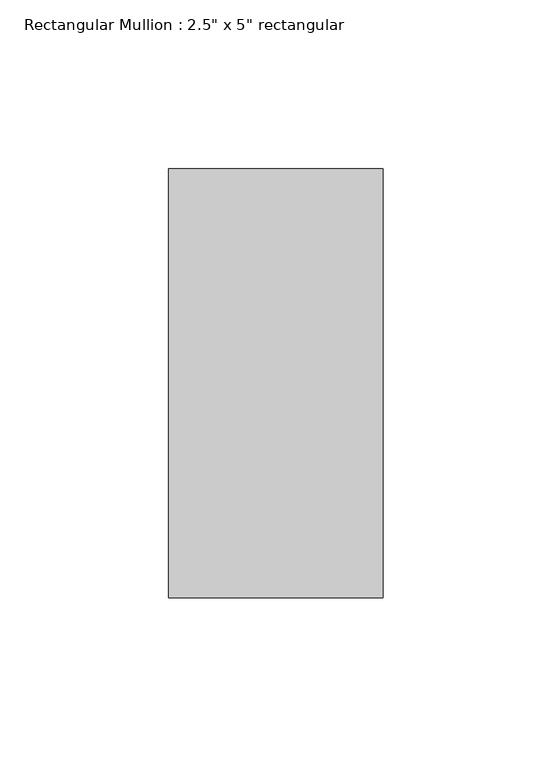
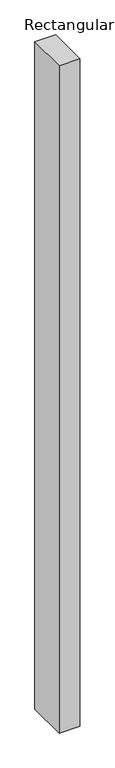
"""IFC4 building model written with IfcOpenShell, lengths in millimetres: member geometry."""

from ifc_helpers import new_model, si_unit, frame, origin, place, context, project, spatial, polyline, outline, extrude, source, transform, mapped, element, save


def member_fbb18fbc(model_context):
    return source(origin(), model_context, "Body", "SweptSolid", [
        extrude(outline(polyline([(0.0, 63.5), (0.0, -63.5), (-63.5, -63.5), (-63.5, 63.5), (0.0, 63.5)])), frame((0.0, 0.0, -2146.3), z_axis=(0.0, 0.0, 1.0), x_axis=(1.0, 0.0, 0.0)), (0.0, 0.0, 1.0), 2146.3),
    ])


if __name__ == "__main__":
    model = new_model("IFC4")
    model_context = context("Model", 3, world=origin())
    ifc_project = project(units=[si_unit("LENGTHUNIT", "METRE", prefix="MILLI")], contexts=[model_context])
    site = spatial("IfcSite", under=ifc_project)
    building = spatial("IfcBuilding", under=site)
    placement = place(None, origin())
    member_shape = member_fbb18fbc(model_context)
    element("IfcMember", 1, ObjectType="Rectangular Mullion : 2.5\" x 5\" rectangular", at=placement, inside=building, context=model_context, shape_type="MappedRepresentation", body=[
        mapped(member_shape, transform((0.0, 0.0, 0.0), x_axis=(1.0, 0.0, 0.0), y_axis=(0.0, 1.0, 0.0), z_axis=(0.0, 0.0, 1.0))),
    ])
    save(model, "model.ifc")

# Revit data of these elements
# Type "Rectangular Mullion : 2.5\" x 5\" rectangular"
#   built-in parameter 1007304 = 0.416667 (stored number, unit not read)
#   built-in parameter 1007301 = 0.104167 (stored number, unit not read)
#   built-in parameter 1007300 = 0.104167 (stored number, unit not read)
# Element 1 (IfcMember, "Rectangular Mullion : 2.5\" x 5\" rectangular")
#   Materials on its faces: "Aluminum"
# Materials
#   "Aluminum": class "Metal", colour RGB 247 247 247, transparency 0, Description = "Aluminum 6061", Cost = 0
